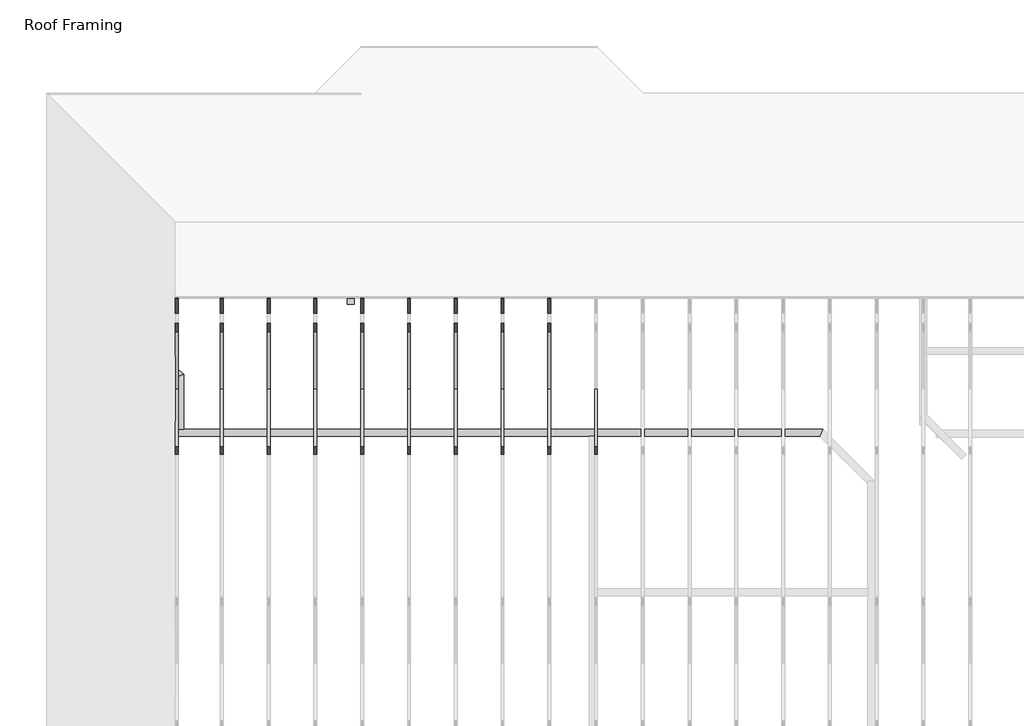
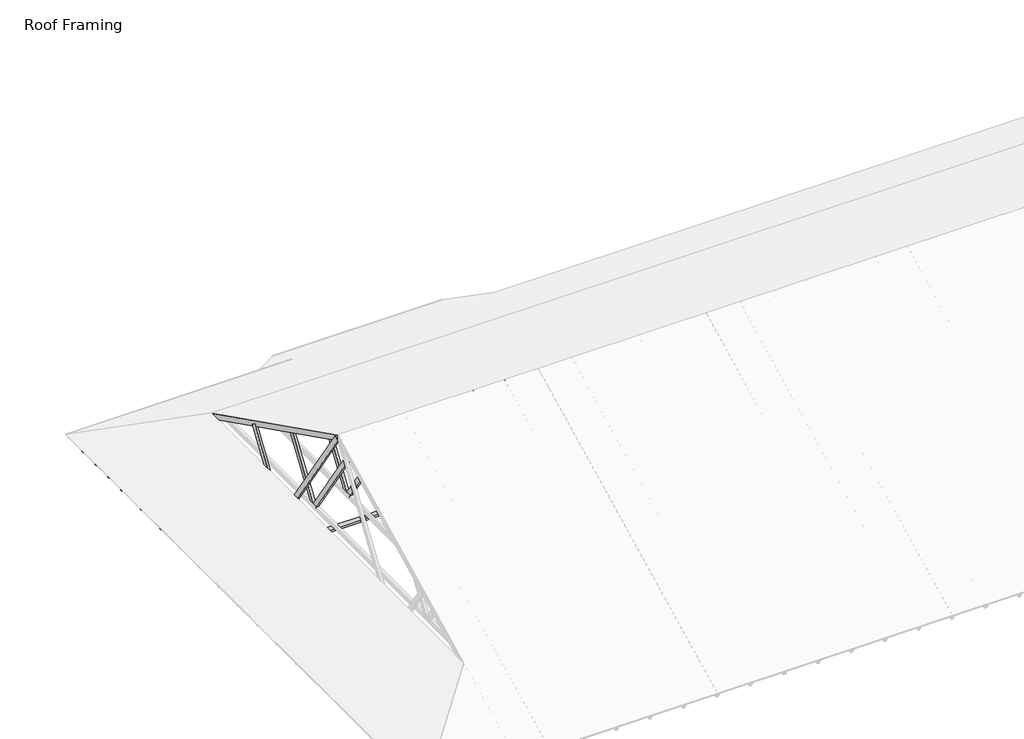
# One storey, part 5 of 7: 46 beams, 19 members.
"""IFC4 building model written with IfcOpenShell, lengths in millimetres."""

import ifcopenshell
import ifcopenshell.guid

model = None  # the IFC model being written
_history = None  # IfcOwnerHistory: only IFC2X3 demands one
_inside = {}  # id of a spatial element -> (the spatial element, [elements in it])
_under = {}  # id of a project, library or spatial element -> (it, [spatial elements below it])
_declared = {}  # id of a project -> (the project, [libraries it declares])
_typed = {}  # id of a type object -> (the type object, [elements of that type])
_made_of = {}  # id of a material, layer set ... -> (it, [elements and type objects made of it])


def new_model(schema):
    """Start an empty IFC model of exactly this schema.

    Asked for "IFC4X3", IfcOpenShell would pick the latest addendum, in which some entities
    have other attributes; the version numbers below select the first issue.
    IFC2X3 requires an IfcOwnerHistory on every rooted entity: one is made here for all.
    """
    global model, _history
    if schema == "IFC4X3":
        model = ifcopenshell.file(schema_version=(4, 3, 0, 0))
    else:
        model = ifcopenshell.file(schema=schema)
    _inside.clear()
    _under.clear()
    _declared.clear()
    _typed.clear()
    _made_of.clear()
    _history = None
    if model.schema == "IFC2X3":
        org = make("IfcOrganization", Name="unknown")
        user = make(
            "IfcPersonAndOrganization",
            ThePerson=make("IfcPerson", FamilyName="unknown"),
            TheOrganization=org,
        )
        app = make(
            "IfcApplication",
            ApplicationDeveloper=org,
            Version="unknown",
            ApplicationFullName="unknown",
            ApplicationIdentifier="unknown",
        )
        _history = make(
            "IfcOwnerHistory",
            OwningUser=user,
            OwningApplication=app,
            ChangeAction="ADDED",
            CreationDate=0,
        )
    return model


def make(cls, **values):
    """One entity of the class cls with the attributes given. An attribute that is None is left unset."""
    return model.create_entity(
        cls, **{name: value for name, value in values.items() if value is not None}
    )


def rooted(cls, **values):
    """An entity with a GlobalId (a new one), such as an element, a storey or a relation."""
    return make(cls, GlobalId=ifcopenshell.guid.new(), OwnerHistory=_history, **values)


def si_unit(unit_type, name, prefix=None):
    """IfcSIUnit, for example si_unit("LENGTHUNIT", "METRE", prefix="MILLI")."""
    return make("IfcSIUnit", UnitType=unit_type, Prefix=prefix, Name=name)


def assignment(units):
    """IfcUnitAssignment: the units of a project."""
    return None if units is None else make("IfcUnitAssignment", Units=units)


def point(xyz):
    """IfcCartesianPoint."""
    return None if xyz is None else make("IfcCartesianPoint", Coordinates=xyz)


def direction(xyz):
    """IfcDirection."""
    return None if xyz is None else make("IfcDirection", DirectionRatios=xyz)


def frame(location, z_axis=None, x_axis=None):
    """IfcAxis2Placement3D, a coordinate frame: its origin and axes. An axis left out is left unset."""
    return make(
        "IfcAxis2Placement3D",
        Location=point(location),
        Axis=direction(z_axis),
        RefDirection=direction(x_axis),
    )


def origin():
    """The frame at (0, 0, 0) with its axes left unset."""
    return frame((0.0, 0.0, 0.0))


def place(relative_to, where):
    """IfcLocalPlacement: puts the frame where relative to a parent placement (None: the world)."""
    return make(
        "IfcLocalPlacement", PlacementRelTo=relative_to, RelativePlacement=where
    )


def context(
    kind, dimensions, precision=None, world=None, true_north=None, identifier=None
):
    """IfcGeometricRepresentationContext, for example the 3D "Model" context."""
    return make(
        "IfcGeometricRepresentationContext",
        ContextIdentifier=identifier,
        ContextType=kind,
        CoordinateSpaceDimension=dimensions,
        Precision=precision,
        WorldCoordinateSystem=world,
        TrueNorth=true_north,
    )


def project(units=None, contexts=None):
    """IfcProject with its units and contexts."""
    return rooted(
        "IfcProject",
        Name="project",
        RepresentationContexts=contexts,
        UnitsInContext=assignment(units),
    )


def spatial(cls, under=None, at=None, **own):
    """A site, building, storey or space (cls), placed at a placement, below another one or the project."""
    s = rooted(cls, ObjectPlacement=at, **own)
    if under is not None:
        _under.setdefault(under.id(), (under, []))[1].append(s)
    return s


def polyline(points):
    """IfcPolyline through the points."""
    return make("IfcPolyline", Points=[point(p) for p in points])


def outline(outer, holes=None, kind="AREA"):
    """IfcArbitraryClosedProfileDef: a profile drawn as a closed curve; with holes, ...WithVoids."""
    if holes is None:
        return make("IfcArbitraryClosedProfileDef", ProfileType=kind, OuterCurve=outer)
    return make(
        "IfcArbitraryProfileDefWithVoids",
        ProfileType=kind,
        OuterCurve=outer,
        InnerCurves=holes,
    )


def extrude(swept, where, along, depth):
    """IfcExtrudedAreaSolid: the profile swept, set in the frame where, extruded along a direction by depth."""
    return make(
        "IfcExtrudedAreaSolid",
        SweptArea=swept,
        Position=where,
        ExtrudedDirection=direction(along),
        Depth=depth,
    )


def shape(context_of_items, identifier, shape_type, items):
    """IfcShapeRepresentation: the items that make up one representation, for example the "Body"."""
    return make(
        "IfcShapeRepresentation",
        ContextOfItems=context_of_items,
        RepresentationIdentifier=identifier,
        RepresentationType=shape_type,
        Items=items,
    )


def source(mapping_origin, context_of_items, identifier, shape_type, items):
    """IfcRepresentationMap: a shape defined once, which mapped items show again and again."""
    return make(
        "IfcRepresentationMap",
        MappingOrigin=mapping_origin,
        MappedRepresentation=shape(context_of_items, identifier, shape_type, items),
    )


def transform(
    local_origin,
    x_axis=None,
    y_axis=None,
    z_axis=None,
    scale=None,
    scale2=None,
    scale3=None,
    uniform=True,
):
    """IfcCartesianTransformationOperator3D, or its non-uniform kind. x_axis, y_axis, z_axis: its Axis1, 2, 3."""
    if uniform:
        return make(
            "IfcCartesianTransformationOperator3D",
            Axis1=direction(x_axis),
            Axis2=direction(y_axis),
            LocalOrigin=point(local_origin),
            Scale=scale,
            Axis3=direction(z_axis),
        )
    return make(
        "IfcCartesianTransformationOperator3DnonUniform",
        Axis1=direction(x_axis),
        Axis2=direction(y_axis),
        LocalOrigin=point(local_origin),
        Scale=scale,
        Axis3=direction(z_axis),
        Scale2=scale2,
        Scale3=scale3,
    )


def mapped(mapping_source, mapping_target):
    """IfcMappedItem: shows the shape of a source again, moved by a transform."""
    return make(
        "IfcMappedItem", MappingSource=mapping_source, MappingTarget=mapping_target
    )


def made_of(thing, what):
    """Note that an element or type object is made of a material, layer set ...; save() writes the relation."""
    if what is not None:
        _made_of.setdefault(what.id(), (what, []))[1].append(thing)
    return thing


def element(
    cls,
    number,
    at=None,
    inside=None,
    cuts=None,
    type_object=None,
    material=None,
    context=None,
    identifier="Body",
    shape_type=None,
    held_by="IfcProductDefinitionShape",
    body=None,
    shapes=None,
    **own,
):
    """One element of the class cls, such as IfcWall. Its Tag is "e" and its number.

    at: its placement. inside: the storey or other place that contains it. cuts: it is an
    opening in that element (IfcRelVoidsElement). A single representation is given by context,
    identifier, shape_type and body (its items); several are given by shapes. held_by: the class
    of the entity that holds the representations. save() writes the other relations.
    """
    e = rooted(cls, Tag="e%d" % number, ObjectPlacement=at, **own)
    if body is not None:
        shapes = [shape(context, identifier, shape_type, body)]
    if shapes is not None:
        e.Representation = make(held_by, Representations=shapes)
    if inside is not None:
        _inside.setdefault(inside.id(), (inside, []))[1].append(e)
    if cuts is not None:
        rooted(
            "IfcRelVoidsElement", RelatingBuildingElement=cuts, RelatedOpeningElement=e
        )
    if type_object is not None:
        _typed.setdefault(type_object.id(), (type_object, []))[1].append(e)
    return made_of(e, material)


def aggregate(whole, parts):
    """IfcRelAggregates: a whole, such as a stair, and the parts it consists of."""
    return rooted("IfcRelAggregates", RelatingObject=whole, RelatedObjects=parts)


def save(model, path):
    """Write the relations noted so far, then the file.

    IfcRelAggregates (storeys below a building ...), IfcRelContainedInSpatialStructure (elements
    in a storey), IfcRelDefinesByType, IfcRelAssociatesMaterial and IfcRelDeclares: one each for
    every whole, place, type object, material and project.
    """
    for whole, parts in _under.values():
        aggregate(whole, parts)
    for where, things in _inside.values():
        rooted(
            "IfcRelContainedInSpatialStructure",
            RelatedElements=things,
            RelatingStructure=where,
        )
    for kind, things in _typed.values():
        rooted("IfcRelDefinesByType", RelatedObjects=things, RelatingType=kind)
    for what, things in _made_of.values():
        rooted("IfcRelAssociatesMaterial", RelatedObjects=things, RelatingMaterial=what)
    for by, libraries in _declared.values():
        rooted("IfcRelDeclares", RelatingContext=by, RelatedDefinitions=libraries)
    model.write(path)


def dimension_lumber_2cac8895(model_context):
    return source(origin(), model_context, "Body", "SweptSolid", [
        extrude(outline(polyline([(1119.2453323, 44.45), (1119.2453323, -44.45), (-1074.7953323, -44.45), (-1074.7953323, 44.45), (1119.2453323, 44.45)])), frame((0.0, 0.0, -19.05), z_axis=(0.0, 0.0, 1.0), x_axis=(1.0, 0.0, 0.0)), (0.0, 0.0, 1.0), 38.1),
    ])


def dimension_lumber_dae2390a(model_context):
    return source(origin(), model_context, "Body", "SweptSolid", [
        extrude(outline(polyline([(120.65, 44.45), (120.65, -44.45), (-3333.75, -44.45), (-3333.75, 44.45), (120.65, 44.45)])), frame((0.0, 0.0, -19.05), z_axis=(0.0, 0.0, 1.0), x_axis=(1.0, 0.0, 0.0)), (0.0, 0.0, 1.0), 38.1),
    ])


def dimension_lumber_0ba03532(model_context):
    return source(origin(), model_context, "Body", "SweptSolid", [
        extrude(outline(polyline([(1590.9128229, 44.45), (1590.9128229, -44.45), (-1571.3871771, -44.45), (-1571.3871771, 44.45), (1590.9128229, 44.45)])), frame((0.0, 0.0, -19.05), z_axis=(0.0, 0.0, 1.0), x_axis=(1.0, 0.0, 0.0)), (0.0, 0.0, 1.0), 38.1),
    ])


def dimension_lumber_2x10_header_exterior_df58e940(model_context):
    return source(origin(), model_context, "Body", "SweptSolid", [
        extrude(outline(polyline([(1646.2375, 19.05), (1646.2375, -19.05), (-1592.2625, -19.05), (-1592.2625, 19.05), (1646.2375, 19.05)])), frame((0.0, 0.0, -117.475), z_axis=(0.0, 0.0, 1.0), x_axis=(1.0, 0.0, 0.0)), (0.0, 0.0, 1.0), 234.95),
    ])


model = new_model("IFC4")

# Units and contexts
model_context = context("Model", 3, world=origin())
ifc_project = project(units=[si_unit("LENGTHUNIT", "METRE", prefix="MILLI")], contexts=[model_context])

# Site, building, storey
site = spatial("IfcSite", under=ifc_project)
building = spatial("IfcBuilding", under=site)
storey = spatial("IfcBuildingStorey", under=building, Name="Roof Framing", Elevation=2768.6)

# Beams
placement = place(None, origin())
element("IfcBeam", 1, ObjectType="Dimension Lumber : Roof Lumbers", at=placement, inside=storey, context=model_context, shape_type="SweptSolid", body=[
    extrude(outline(polyline([(-5032.8152251, 251.1959053), (-5032.8152251, 213.0959053), (-6240.9027251, 213.0959053), (-6240.9027251, 251.1959053), (-5032.8152251, 251.1959053)])), frame((0.0, 0.0, 2768.6), z_axis=(0.0, 0.0, 1.0), x_axis=(1.0, 0.0, 0.0)), (0.0, 0.0, 1.0), 88.9),
    extrude(outline(polyline([(2768.6, -5032.8152251), (2857.5, -5032.8152251), (2857.5, -6064.1385305), (2769.1179027, -6240.9027251), (2768.6, -6240.9027251), (2768.6, -5032.8152251)])), frame((0.0, 213.0959053, 0.0), z_axis=(0.0, 1.0, 0.0), x_axis=(0.0, 0.0, 1.0)), (0.0, 0.0, 1.0), 38.1),
])
element("IfcBeam", 2, ObjectType="Dimension Lumber : Roof Lumbers", at=placement, inside=storey, context=model_context, shape_type="SweptSolid", body=[
    extrude(outline(polyline([(-5032.8152251, 860.7959053), (-5032.8152251, 822.6959053), (-6240.9027251, 822.6959053), (-6240.9027251, 860.7959053), (-5032.8152251, 860.7959053)])), frame((0.0, 0.0, 2768.6), z_axis=(0.0, 0.0, 1.0), x_axis=(1.0, 0.0, 0.0)), (0.0, 0.0, 1.0), 88.9),
    extrude(outline(polyline([(2768.6, -5032.8152251), (2857.5, -5032.8152251), (2857.5, -6064.1385305), (2769.1179027, -6240.9027251), (2768.6, -6240.9027251), (2768.6, -5032.8152251)])), frame((0.0, 822.6959053, 0.0), z_axis=(0.0, 1.0, 0.0), x_axis=(0.0, 0.0, 1.0)), (0.0, 0.0, 1.0), 38.1),
])
element("IfcBeam", 3, ObjectType="Dimension Lumber : Roof Lumbers", at=placement, inside=storey, context=model_context, shape_type="SweptSolid", body=[
    extrude(outline(polyline([(-5032.8152251, 1470.3959053), (-5032.8152251, 1432.2959053), (-6240.9027251, 1432.2959053), (-6240.9027251, 1470.3959053), (-5032.8152251, 1470.3959053)])), frame((0.0, 0.0, 2768.6), z_axis=(0.0, 0.0, 1.0), x_axis=(1.0, 0.0, 0.0)), (0.0, 0.0, 1.0), 88.9),
    extrude(outline(polyline([(2768.6, -5032.8152251), (2857.5, -5032.8152251), (2857.5, -6064.1385305), (2769.1179027, -6240.9027251), (2768.6, -6240.9027251), (2768.6, -5032.8152251)])), frame((0.0, 1432.2959053, 0.0), z_axis=(0.0, 1.0, 0.0), x_axis=(0.0, 0.0, 1.0)), (0.0, 0.0, 1.0), 38.1),
])
element("IfcBeam", 4, ObjectType="Dimension Lumber : Roof Lumbers", at=placement, inside=storey, context=model_context, shape_type="SweptSolid", body=[
    extrude(outline(polyline([(-5032.8152251, 2079.9959053), (-5032.8152251, 2041.8959053), (-6240.9027251, 2041.8959053), (-6240.9027251, 2079.9959053), (-5032.8152251, 2079.9959053)])), frame((0.0, 0.0, 2768.6), z_axis=(0.0, 0.0, 1.0), x_axis=(1.0, 0.0, 0.0)), (0.0, 0.0, 1.0), 88.9),
    extrude(outline(polyline([(2768.6, -5032.8152251), (2857.5, -5032.8152251), (2857.5, -6064.1385305), (2769.1179027, -6240.9027251), (2768.6, -6240.9027251), (2768.6, -5032.8152251)])), frame((0.0, 2041.8959053, 0.0), z_axis=(0.0, 1.0, 0.0), x_axis=(0.0, 0.0, 1.0)), (0.0, 0.0, 1.0), 38.1),
])
element("IfcBeam", 5, ObjectType="Dimension Lumber : Roof Lumbers", at=placement, inside=storey, context=model_context, shape_type="SweptSolid", body=[
    extrude(outline(polyline([(-5032.8152251, 2689.5959053), (-5032.8152251, 2651.4959053), (-6240.9027251, 2651.4959053), (-6240.9027251, 2689.5959053), (-5032.8152251, 2689.5959053)])), frame((0.0, 0.0, 2768.6), z_axis=(0.0, 0.0, 1.0), x_axis=(1.0, 0.0, 0.0)), (0.0, 0.0, 1.0), 88.9),
    extrude(outline(polyline([(2768.6, -5032.8152251), (2857.5, -5032.8152251), (2857.5, -6064.1385305), (2769.1179027, -6240.9027251), (2768.6, -6240.9027251), (2768.6, -5032.8152251)])), frame((0.0, 2651.4959053, 0.0), z_axis=(0.0, 1.0, 0.0), x_axis=(0.0, 0.0, 1.0)), (0.0, 0.0, 1.0), 38.1),
])
element("IfcBeam", 6, ObjectType="Dimension Lumber : Roof Lumbers", at=placement, inside=storey, context=model_context, shape_type="SweptSolid", body=[
    extrude(outline(polyline([(-5032.8152251, 3299.1959053), (-5032.8152251, 3261.0959053), (-6240.9027251, 3261.0959053), (-6240.9027251, 3299.1959053), (-5032.8152251, 3299.1959053)])), frame((0.0, 0.0, 2768.6), z_axis=(0.0, 0.0, 1.0), x_axis=(1.0, 0.0, 0.0)), (0.0, 0.0, 1.0), 88.9),
    extrude(outline(polyline([(2768.6, -5032.8152251), (2857.5, -5032.8152251), (2857.5, -6064.1385305), (2769.1179027, -6240.9027251), (2768.6, -6240.9027251), (2768.6, -5032.8152251)])), frame((0.0, 3261.0959053, 0.0), z_axis=(0.0, 1.0, 0.0), x_axis=(0.0, 0.0, 1.0)), (0.0, 0.0, 1.0), 38.1),
])
element("IfcBeam", 7, ObjectType="Dimension Lumber : Top Supporting Lumbers", at=placement, inside=storey, context=model_context, shape_type="SweptSolid", body=[
    extrude(outline(polyline([(-133.4609188, 5097.8334053), (-133.4609188, 5008.9334053), (-2129.5888108, 5008.9334053), (-2129.5888108, 5097.8334053), (-133.4609188, 5097.8334053)])), frame((0.0, 0.0, 2425.7), z_axis=(0.0, 0.0, 1.0), x_axis=(1.0, 0.0, 0.0)), (0.0, 0.0, 1.0), 38.1),
    extrude(outline(polyline([(-181.7263108, 5008.9334053), (-2129.5888108, 5008.9334053), (-2129.5888108, 5097.8334053), (-144.9027251, 5097.8334053), (-181.7263108, 5008.9334053)])), frame((0.0, 0.0, 2425.7), z_axis=(0.0, 0.0, 1.0), x_axis=(1.0, 0.0, 0.0)), (0.0, 0.0, 1.0), 38.1),
    extrude(outline(polyline([(-181.7263108, 5008.9334053), (-1936.8791394, 5008.9334053), (-1973.7027251, 5097.8334053), (-144.9027251, 5097.8334053), (-181.7263108, 5008.9334053)])), frame((0.0, 0.0, 2425.7), z_axis=(0.0, 0.0, 1.0), x_axis=(1.0, 0.0, 0.0)), (0.0, 0.0, 1.0), 38.1),
])
element("IfcBeam", 8, ObjectType="Dimension Lumber : Top Supporting Lumbers", at=placement, inside=storey, context=model_context, shape_type="SweptSolid", body=[
    extrude(outline(polyline([(-136.9652251, 5097.8334053), (-136.9652251, 5008.9334053), (-1984.8152251, 5008.9334053), (-1984.8152251, 5097.8334053), (-136.9652251, 5097.8334053)])), frame((0.0, 0.0, 2387.6), z_axis=(0.0, 0.0, 1.0), x_axis=(1.0, 0.0, 0.0)), (0.0, 0.0, 1.0), 38.1),
    extrude(outline(polyline([(-136.9652251, 5097.8334053), (-136.9652251, 5008.9334053), (-1936.8791394, 5008.9334053), (-1973.7027251, 5097.8334053), (-136.9652251, 5097.8334053)])), frame((0.0, 0.0, 2387.6), z_axis=(0.0, 0.0, 1.0), x_axis=(1.0, 0.0, 0.0)), (0.0, 0.0, 1.0), 38.1),
    extrude(outline(polyline([(-181.7263108, 5008.9334053), (-1936.8791394, 5008.9334053), (-1973.7027251, 5097.8334053), (-144.9027251, 5097.8334053), (-181.7263108, 5008.9334053)])), frame((0.0, 0.0, 2387.6), z_axis=(0.0, 0.0, 1.0), x_axis=(1.0, 0.0, 0.0)), (0.0, 0.0, 1.0), 38.1),
])
element("IfcBeam", 9, ObjectType="Dimension Lumber : Top Supporting Lumbers", at=placement, inside=storey, context=model_context, shape_type="SweptSolid", body=[
    extrude(outline(polyline([(-2584.7694335, 4361.0431112), (-2647.6312264, 4423.904904), (-1974.0218287, 5097.5143017), (-1911.1600358, 5034.6525089), (-2584.7694335, 4361.0431112)])), frame((0.0, 0.0, 2425.7), z_axis=(0.0, 0.0, 1.0), x_axis=(1.0, 0.0, 0.0)), (0.0, 0.0, 1.0), 38.1),
    extrude(outline(polyline([(-2584.7694335, 4361.0431112), (-2647.6312264, 4423.904904), (-1974.0218287, 5097.5143017), (-1973.2514445, 5096.7439175), (-1936.8791394, 5008.9334053), (-2584.7694335, 4361.0431112)])), frame((0.0, 0.0, 2425.7), z_axis=(0.0, 0.0, 1.0), x_axis=(1.0, 0.0, 0.0)), (0.0, 0.0, 1.0), 38.1),
    extrude(outline(polyline([(-2623.0597276, 4399.3334053), (-2647.6312264, 4423.904904), (-1974.0218287, 5097.5143017), (-1973.2514445, 5096.7439175), (-1936.8791394, 5008.9334053), (-2546.4791394, 4399.3334053), (-2623.0597276, 4399.3334053)])), frame((0.0, 0.0, 2425.7), z_axis=(0.0, 0.0, 1.0), x_axis=(1.0, 0.0, 0.0)), (0.0, 0.0, 1.0), 38.1),
    extrude(outline(polyline([(-2621.4027251, 4450.1334053), (-1974.0218287, 5097.5143017), (-1973.2514445, 5096.7439175), (-1936.8791394, 5008.9334053), (-2546.4791394, 4399.3334053), (-2621.4027251, 4399.3334053), (-2621.4027251, 4450.1334053)])), frame((0.0, 0.0, 2425.7), z_axis=(0.0, 0.0, 1.0), x_axis=(1.0, 0.0, 0.0)), (0.0, 0.0, 1.0), 38.1),
])
element("IfcBeam", 10, ObjectType="Dimension Lumber : Top Supporting Lumbers", at=placement, inside=storey, context=model_context, shape_type="SweptSolid", body=[
    extrude(outline(polyline([(-1969.4575758, 5102.0785546), (-1906.595783, 5039.2167618), (-2584.7694335, 4361.0431112), (-2647.6312264, 4423.904904), (-1969.4575758, 5102.0785546)])), frame((0.0, 0.0, 2387.6), z_axis=(0.0, 0.0, 1.0), x_axis=(1.0, 0.0, 0.0)), (0.0, 0.0, 1.0), 38.1),
    extrude(outline(polyline([(-1936.8791394, 5008.9334053), (-2584.7694335, 4361.0431112), (-2647.6312264, 4423.904904), (-1973.7027251, 5097.8334053), (-1936.8791394, 5008.9334053)])), frame((0.0, 0.0, 2387.6), z_axis=(0.0, 0.0, 1.0), x_axis=(1.0, 0.0, 0.0)), (0.0, 0.0, 1.0), 38.1),
    extrude(outline(polyline([(-1936.8791394, 5008.9334053), (-2546.4791394, 4399.3334053), (-2623.0597276, 4399.3334053), (-2647.6312264, 4423.904904), (-1973.7027251, 5097.8334053), (-1936.8791394, 5008.9334053)])), frame((0.0, 0.0, 2387.6), z_axis=(0.0, 0.0, 1.0), x_axis=(1.0, 0.0, 0.0)), (0.0, 0.0, 1.0), 38.1),
    extrude(outline(polyline([(-1936.8791394, 5008.9334053), (-2546.4791394, 4399.3334053), (-2621.4027251, 4399.3334053), (-2621.4027251, 4450.1334053), (-1973.7027251, 5097.8334053), (-1936.8791394, 5008.9334053)])), frame((0.0, 0.0, 2387.6), z_axis=(0.0, 0.0, 1.0), x_axis=(1.0, 0.0, 0.0)), (0.0, 0.0, 1.0), 38.1),
])
element("IfcBeam", 11, ObjectType="Dimension Lumber : Top Supporting Lumbers", at=placement, inside=storey, context=model_context, shape_type="SweptSolid", body=[
    extrude(outline(polyline([(-5544.0627459, 1818.4935621), (-5576.4196998, 1729.5935621), (-6152.0027251, 1729.5935621), (-6152.0027251, 1818.4935621), (-5544.0627459, 1818.4935621)])), frame((0.0, 0.0, 2692.4), z_axis=(0.0, 0.0, 1.0), x_axis=(1.0, 0.0, 0.0)), (0.0, 0.0, 1.0), 38.1),
])
element("IfcBeam", 12, ObjectType="Dimension Lumber : Top Supporting Lumbers", at=placement, inside=storey, context=model_context, shape_type="SweptSolid", body=[
    extrude(outline(polyline([(-4923.2263621, 1297.5499814), (-5012.1263621, 1256.0952306), (-5576.4196998, 1729.5935621), (-5544.0627459, 1818.4935621), (-4923.2263621, 1297.5499814)])), frame((0.0, 0.0, 2692.4), z_axis=(0.0, 0.0, 1.0), x_axis=(1.0, 0.0, 0.0)), (0.0, 0.0, 1.0), 38.1),
])
element("IfcBeam", 13, ObjectType="Dimension Lumber : Top Supporting Lumbers", at=placement, inside=storey, context=model_context, shape_type="SweptSolid", body=[
    extrude(outline(polyline([(-4923.2263621, 578.2209053), (-5012.1263621, 578.2209053), (-5012.1263621, 1256.0952306), (-4923.2263621, 1297.5499814), (-4923.2263621, 578.2209053)])), frame((0.0, 0.0, 2692.4), z_axis=(0.0, 0.0, 1.0), x_axis=(1.0, 0.0, 0.0)), (0.0, 0.0, 1.0), 38.1),
])
element("IfcBeam", 14, ObjectType="Dimension Lumber : Top Supporting Lumbers", at=placement, inside=storey, context=model_context, shape_type="SweptSolid", body=[
    extrude(outline(polyline([(3409.5097749, 578.2209053), (3372.6861892, 489.3209053), (-6152.0027251, 489.3209053), (-6152.0027251, 578.2209053), (3409.5097749, 578.2209053)])), frame((0.0, 0.0, 2692.4), z_axis=(0.0, 0.0, 1.0), x_axis=(1.0, 0.0, 0.0)), (0.0, 0.0, 1.0), 38.1),
])
dimension_lumber_shape = dimension_lumber_2cac8895(model_context)
element("IfcBeam", 15, ObjectType="Dimension Lumber : Top Supporting Lumbers", at=placement, inside=storey, context=model_context, shape_type="MappedRepresentation", body=[
    mapped(dimension_lumber_shape, transform((-2742.0527251, 3324.538073, 2711.45), x_axis=(0.0, -1.0, 0.0), y_axis=(1.0, 0.0, 0.0), z_axis=(0.0, 0.0, 1.0))),
])
dimension_lumber_2_shape = dimension_lumber_dae2390a(model_context)
element("IfcBeam", 16, ObjectType="Dimension Lumber : Top Supporting Lumbers", at=placement, inside=storey, context=model_context, shape_type="MappedRepresentation", body=[
    mapped(dimension_lumber_2_shape, transform((-2818.2527251, 4443.7834053, 2711.45), x_axis=(1.0, 0.0, 0.0), y_axis=(0.0, 1.0, 0.0), z_axis=(0.0, 0.0, 1.0))),
])
dimension_lumber_3_shape = dimension_lumber_0ba03532(model_context)
element("IfcBeam", 17, ObjectType="Dimension Lumber : Top Supporting Lumbers", at=placement, inside=storey, context=model_context, shape_type="MappedRepresentation", body=[
    mapped(dimension_lumber_3_shape, transform((-1088.115548, 4443.7834053, 2438.796875), x_axis=(1.0, 0.0, 0.0), y_axis=(0.0, 1.0, 0.0), z_axis=(0.0, 0.0, 1.0))),
])
dimension_lumber_2x10_header_exterior_shape = dimension_lumber_2x10_header_exterior_df58e940(model_context)
element("IfcBeam", 18, ObjectType="Dimension Lumber : 2x10 Header Exterior", at=placement, inside=storey, context=model_context, shape_type="MappedRepresentation", body=[
    mapped(dimension_lumber_2x10_header_exterior_shape, transform((-1105.3402251, 4469.1834053, 2651.125), x_axis=(1.0, 0.0, 0.0), y_axis=(0.0, 1.0, 0.0), z_axis=(0.0, 0.0, 1.0))),
])
element("IfcBeam", 19, ObjectType="Dimension Lumber : 2x10 Header Exterior", at=placement, inside=storey, context=model_context, shape_type="MappedRepresentation", body=[
    mapped(dimension_lumber_2x10_header_exterior_shape, transform((-1105.3402251, 4418.3834053, 2651.125), x_axis=(1.0, 0.0, 0.0), y_axis=(0.0, 1.0, 0.0), z_axis=(0.0, 0.0, 1.0))),
])
element("IfcBeam", 20, ObjectType="Dimension Lumber : 2x4 Blocking", at=placement, inside=storey, context=model_context, shape_type="SweptSolid", body=[
    extrude(outline(polyline([(-6671.1152251, 2041.8959053), (-6671.1152251, 2079.9959053), (-6290.1152251, 2079.9959053), (-6290.1152251, 2041.8959053), (-6671.1152251, 2041.8959053)])), frame((0.0, 0.0, 2564.60625), z_axis=(0.0, 0.0, 1.0), x_axis=(1.0, 0.0, 0.0)), (0.0, 0.0, 1.0), 88.9),
    extrude(outline(polyline([(2564.60625, -6649.9260305), (2564.60625, -6290.1152251), (2653.50625, -6290.1152251), (2653.50625, -6472.1260305), (2564.60625, -6649.9260305)])), frame((0.0, 2041.8959053, 0.0), z_axis=(0.0, 1.0, 0.0), x_axis=(0.0, 0.0, 1.0)), (0.0, 0.0, 1.0), 38.1),
])
element("IfcBeam", 21, ObjectType="Dimension Lumber : 2x4 Blocking", at=placement, inside=storey, context=model_context, shape_type="SweptSolid", body=[
    extrude(outline(polyline([(-6671.1152251, 2651.4959053), (-6671.1152251, 2689.5959053), (-6290.1152251, 2689.5959053), (-6290.1152251, 2651.4959053), (-6671.1152251, 2651.4959053)])), frame((0.0, 0.0, 2564.60625), z_axis=(0.0, 0.0, 1.0), x_axis=(1.0, 0.0, 0.0)), (0.0, 0.0, 1.0), 88.9),
    extrude(outline(polyline([(2564.60625, -6649.9260305), (2564.60625, -6290.1152251), (2653.50625, -6290.1152251), (2653.50625, -6472.1260305), (2564.60625, -6649.9260305)])), frame((0.0, 2651.4959053, 0.0), z_axis=(0.0, 1.0, 0.0), x_axis=(0.0, 0.0, 1.0)), (0.0, 0.0, 1.0), 38.1),
])
element("IfcBeam", 22, ObjectType="Dimension Lumber : 2x4 Blocking", at=placement, inside=storey, context=model_context, shape_type="SweptSolid", body=[
    extrude(outline(polyline([(-6671.1152251, 3261.0959053), (-6671.1152251, 3299.1959053), (-6290.1152251, 3299.1959053), (-6290.1152251, 3261.0959053), (-6671.1152251, 3261.0959053)])), frame((0.0, 0.0, 2564.60625), z_axis=(0.0, 0.0, 1.0), x_axis=(1.0, 0.0, 0.0)), (0.0, 0.0, 1.0), 88.9),
    extrude(outline(polyline([(2564.60625, -6649.9260305), (2564.60625, -6290.1152251), (2653.50625, -6290.1152251), (2653.50625, -6472.1260305), (2564.60625, -6649.9260305)])), frame((0.0, 3261.0959053, 0.0), z_axis=(0.0, 1.0, 0.0), x_axis=(0.0, 0.0, 1.0)), (0.0, 0.0, 1.0), 38.1),
])
element("IfcBeam", 23, ObjectType="Dimension Lumber : 2x4 Blocking", at=placement, inside=storey, context=model_context, shape_type="SweptSolid", body=[
    extrude(outline(polyline([(-175.0652251, 5147.0459053), (-175.0652251, 5528.0459053), (-136.9652251, 5528.0459053), (-136.9652251, 5147.0459053), (-175.0652251, 5147.0459053)])), frame((0.0, 0.0, 2259.80625), z_axis=(0.0, 0.0, 1.0), x_axis=(1.0, 0.0, 0.0)), (0.0, 0.0, 1.0), 88.9),
    extrude(outline(polyline([(5147.0459053, 2348.70625), (5329.0567107, 2348.70625), (5506.8567107, 2259.80625), (5147.0459053, 2259.80625), (5147.0459053, 2348.70625)])), frame((-175.0652251, 0.0, 0.0), z_axis=(1.0, 0.0, 0.0), x_axis=(0.0, 1.0, 0.0)), (0.0, 0.0, 1.0), 38.1),
])
element("IfcBeam", 24, ObjectType="Dimension Lumber : 2x4 Blocking", at=placement, inside=storey, context=model_context, shape_type="SweptSolid", body=[
    extrude(outline(polyline([(-784.6652251, 5147.0459053), (-784.6652251, 5528.0459053), (-746.5652251, 5528.0459053), (-746.5652251, 5147.0459053), (-784.6652251, 5147.0459053)])), frame((0.0, 0.0, 2259.80625), z_axis=(0.0, 0.0, 1.0), x_axis=(1.0, 0.0, 0.0)), (0.0, 0.0, 1.0), 88.9),
    extrude(outline(polyline([(5147.0459053, 2348.70625), (5329.0567107, 2348.70625), (5506.8567107, 2259.80625), (5147.0459053, 2259.80625), (5147.0459053, 2348.70625)])), frame((-784.6652251, 0.0, 0.0), z_axis=(1.0, 0.0, 0.0), x_axis=(0.0, 1.0, 0.0)), (0.0, 0.0, 1.0), 38.1),
])
element("IfcBeam", 25, ObjectType="Dimension Lumber : 2x4 Blocking", at=placement, inside=storey, context=model_context, shape_type="SweptSolid", body=[
    extrude(outline(polyline([(-1394.2652251, 5147.0459053), (-1394.2652251, 5528.0459053), (-1356.1652251, 5528.0459053), (-1356.1652251, 5147.0459053), (-1394.2652251, 5147.0459053)])), frame((0.0, 0.0, 2259.80625), z_axis=(0.0, 0.0, 1.0), x_axis=(1.0, 0.0, 0.0)), (0.0, 0.0, 1.0), 88.9),
    extrude(outline(polyline([(5147.0459053, 2348.70625), (5329.0567107, 2348.70625), (5506.8567107, 2259.80625), (5147.0459053, 2259.80625), (5147.0459053, 2348.70625)])), frame((-1394.2652251, 0.0, 0.0), z_axis=(1.0, 0.0, 0.0), x_axis=(0.0, 1.0, 0.0)), (0.0, 0.0, 1.0), 38.1),
])
element("IfcBeam", 26, ObjectType="Dimension Lumber : 2x4 Blocking", at=placement, inside=storey, context=model_context, shape_type="SweptSolid", body=[
    extrude(outline(polyline([(-2003.8652251, 5147.0459053), (-2003.8652251, 5528.0459053), (-1965.7652251, 5528.0459053), (-1965.7652251, 5147.0459053), (-2003.8652251, 5147.0459053)])), frame((0.0, 0.0, 2259.80625), z_axis=(0.0, 0.0, 1.0), x_axis=(1.0, 0.0, 0.0)), (0.0, 0.0, 1.0), 88.9),
    extrude(outline(polyline([(5147.0459053, 2348.70625), (5329.0567107, 2348.70625), (5506.8567107, 2259.80625), (5147.0459053, 2259.80625), (5147.0459053, 2348.70625)])), frame((-2003.8652251, 0.0, 0.0), z_axis=(1.0, 0.0, 0.0), x_axis=(0.0, 1.0, 0.0)), (0.0, 0.0, 1.0), 38.1),
])
element("IfcBeam", 27, ObjectType="Dimension Lumber : 2x4 Blocking", at=placement, inside=storey, context=model_context, shape_type="SweptSolid", body=[
    extrude(outline(polyline([(-2613.4652251, 5147.0459053), (-2613.4652251, 5528.0459053), (-2575.3652251, 5528.0459053), (-2575.3652251, 5147.0459053), (-2613.4652251, 5147.0459053)])), frame((0.0, 0.0, 2259.80625), z_axis=(0.0, 0.0, 1.0), x_axis=(1.0, 0.0, 0.0)), (0.0, 0.0, 1.0), 88.9),
    extrude(outline(polyline([(5147.0459053, 2348.70625), (5329.0567107, 2348.70625), (5506.8567107, 2259.80625), (5147.0459053, 2259.80625), (5147.0459053, 2348.70625)])), frame((-2613.4652251, 0.0, 0.0), z_axis=(1.0, 0.0, 0.0), x_axis=(0.0, 1.0, 0.0)), (0.0, 0.0, 1.0), 38.1),
])
element("IfcBeam", 28, ObjectType="Dimension Lumber : 2x4 Blocking", at=placement, inside=storey, context=model_context, shape_type="SweptSolid", body=[
    extrude(outline(polyline([(-3184.9652251, 4918.4459053), (-3184.9652251, 4537.4459053), (-3223.0652251, 4537.4459053), (-3223.0652251, 4918.4459053), (-3184.9652251, 4918.4459053)])), frame((0.0, 0.0, 2564.60625), z_axis=(0.0, 0.0, 1.0), x_axis=(1.0, 0.0, 0.0)), (0.0, 0.0, 1.0), 88.9),
    extrude(outline(polyline([(4897.2567107, 2564.60625), (4537.4459053, 2564.60625), (4537.4459053, 2653.50625), (4719.4567107, 2653.50625), (4897.2567107, 2564.60625)])), frame((-3223.0652251, 0.0, 0.0), z_axis=(1.0, 0.0, 0.0), x_axis=(0.0, 1.0, 0.0)), (0.0, 0.0, 1.0), 38.1),
])
element("IfcBeam", 29, ObjectType="Dimension Lumber : 2x4 Blocking", at=placement, inside=storey, context=model_context, shape_type="SweptSolid", body=[
    extrude(outline(polyline([(-3794.5652251, 4918.4459053), (-3794.5652251, 4537.4459053), (-3832.6652251, 4537.4459053), (-3832.6652251, 4918.4459053), (-3794.5652251, 4918.4459053)])), frame((0.0, 0.0, 2564.60625), z_axis=(0.0, 0.0, 1.0), x_axis=(1.0, 0.0, 0.0)), (0.0, 0.0, 1.0), 88.9),
    extrude(outline(polyline([(4897.2567107, 2564.60625), (4537.4459053, 2564.60625), (4537.4459053, 2653.50625), (4719.4567107, 2653.50625), (4897.2567107, 2564.60625)])), frame((-3832.6652251, 0.0, 0.0), z_axis=(1.0, 0.0, 0.0), x_axis=(0.0, 1.0, 0.0)), (0.0, 0.0, 1.0), 38.1),
])
element("IfcBeam", 30, ObjectType="Dimension Lumber : 2x4 Blocking", at=placement, inside=storey, context=model_context, shape_type="SweptSolid", body=[
    extrude(outline(polyline([(-4404.1652251, 4918.4459053), (-4404.1652251, 4537.4459053), (-4442.2652251, 4537.4459053), (-4442.2652251, 4918.4459053), (-4404.1652251, 4918.4459053)])), frame((0.0, 0.0, 2564.60625), z_axis=(0.0, 0.0, 1.0), x_axis=(1.0, 0.0, 0.0)), (0.0, 0.0, 1.0), 88.9),
    extrude(outline(polyline([(4897.2567107, 2564.60625), (4537.4459053, 2564.60625), (4537.4459053, 2653.50625), (4719.4567107, 2653.50625), (4897.2567107, 2564.60625)])), frame((-4442.2652251, 0.0, 0.0), z_axis=(1.0, 0.0, 0.0), x_axis=(0.0, 1.0, 0.0)), (0.0, 0.0, 1.0), 38.1),
])
element("IfcBeam", 31, ObjectType="Dimension Lumber : 2x4 Blocking", at=placement, inside=storey, context=model_context, shape_type="SweptSolid", body=[
    extrude(outline(polyline([(-5032.8152251, 4537.4459053), (-5032.8152251, 4918.4459053), (-4994.7152251, 4918.4459053), (-4994.7152251, 4537.4459053), (-5032.8152251, 4537.4459053)])), frame((0.0, 0.0, 2564.60625), z_axis=(0.0, 0.0, 1.0), x_axis=(1.0, 0.0, 0.0)), (0.0, 0.0, 1.0), 88.9),
    extrude(outline(polyline([(4537.4459053, 2653.50625), (4719.4567107, 2653.50625), (4897.2567107, 2564.60625), (4537.4459053, 2564.60625), (4537.4459053, 2653.50625)])), frame((-5032.8152251, 0.0, 0.0), z_axis=(1.0, 0.0, 0.0), x_axis=(0.0, 1.0, 0.0)), (0.0, 0.0, 1.0), 38.1),
])
element("IfcBeam", 32, ObjectType="Dimension Lumber : 2x4 Blocking", at=placement, inside=storey, context=model_context, shape_type="SweptSolid", body=[
    extrude(outline(polyline([(-5458.2652251, 4537.4459053), (-5458.2652251, 4918.4459053), (-5420.1652251, 4918.4459053), (-5420.1652251, 4537.4459053), (-5458.2652251, 4537.4459053)])), frame((0.0, 0.0, 2564.60625), z_axis=(0.0, 0.0, 1.0), x_axis=(1.0, 0.0, 0.0)), (0.0, 0.0, 1.0), 88.9),
    extrude(outline(polyline([(4537.4459053, 2653.50625), (4719.4567107, 2653.50625), (4897.2567107, 2564.60625), (4537.4459053, 2564.60625), (4537.4459053, 2653.50625)])), frame((-5458.2652251, 0.0, 0.0), z_axis=(1.0, 0.0, 0.0), x_axis=(0.0, 1.0, 0.0)), (0.0, 0.0, 1.0), 38.1),
])
element("IfcBeam", 33, ObjectType="Dimension Lumber : 2x4 Blocking", at=placement, inside=storey, context=model_context, shape_type="SweptSolid", body=[
    extrude(outline(polyline([(-5864.6652251, 4537.4459053), (-5864.6652251, 4918.4459053), (-5826.5652251, 4918.4459053), (-5826.5652251, 4537.4459053), (-5864.6652251, 4537.4459053)])), frame((0.0, 0.0, 2564.60625), z_axis=(0.0, 0.0, 1.0), x_axis=(1.0, 0.0, 0.0)), (0.0, 0.0, 1.0), 88.9),
    extrude(outline(polyline([(4537.4459053, 2653.50625), (4719.4567107, 2653.50625), (4897.2567107, 2564.60625), (4537.4459053, 2564.60625), (4537.4459053, 2653.50625)])), frame((-5864.6652251, 0.0, 0.0), z_axis=(1.0, 0.0, 0.0), x_axis=(0.0, 1.0, 0.0)), (0.0, 0.0, 1.0), 38.1),
])
element("IfcBeam", 34, ObjectType="Dimension Lumber : 2x4 Blocking", at=placement, inside=storey, context=model_context, shape_type="SweptSolid", body=[
    extrude(outline(polyline([(-6271.0652251, 4537.4459053), (-6271.0652251, 4918.4459053), (-6232.9652251, 4918.4459053), (-6232.9652251, 4537.4459053), (-6271.0652251, 4537.4459053)])), frame((0.0, 0.0, 2564.60625), z_axis=(0.0, 0.0, 1.0), x_axis=(1.0, 0.0, 0.0)), (0.0, 0.0, 1.0), 88.9),
    extrude(outline(polyline([(4537.4459053, 2653.50625), (4719.4567107, 2653.50625), (4897.2567107, 2564.60625), (4537.4459053, 2564.60625), (4537.4459053, 2653.50625)])), frame((-6271.0652251, 0.0, 0.0), z_axis=(1.0, 0.0, 0.0), x_axis=(0.0, 1.0, 0.0)), (0.0, 0.0, 1.0), 38.1),
])
element("IfcBeam", 35, ObjectType="Dimension Lumber : 2x4 Blocking", at=placement, inside=storey, context=model_context, shape_type="SweptSolid", body=[
    extrude(outline(polyline([(-6671.1152251, 3667.4959053), (-6671.1152251, 3705.5959053), (-6290.1152251, 3705.5959053), (-6290.1152251, 3667.4959053), (-6671.1152251, 3667.4959053)])), frame((0.0, 0.0, 2564.60625), z_axis=(0.0, 0.0, 1.0), x_axis=(1.0, 0.0, 0.0)), (0.0, 0.0, 1.0), 88.9),
    extrude(outline(polyline([(2564.60625, -6649.9260305), (2564.60625, -6290.1152251), (2653.50625, -6290.1152251), (2653.50625, -6472.1260305), (2564.60625, -6649.9260305)])), frame((0.0, 3667.4959053, 0.0), z_axis=(0.0, 1.0, 0.0), x_axis=(0.0, 0.0, 1.0)), (0.0, 0.0, 1.0), 38.1),
])
element("IfcBeam", 36, ObjectType="Dimension Lumber : 2x4 Blocking", at=placement, inside=storey, context=model_context, shape_type="SweptSolid", body=[
    extrude(outline(polyline([(-6671.1152251, 4073.8959053), (-6671.1152251, 4111.9959053), (-6290.1152251, 4111.9959053), (-6290.1152251, 4073.8959053), (-6671.1152251, 4073.8959053)])), frame((0.0, 0.0, 2564.60625), z_axis=(0.0, 0.0, 1.0), x_axis=(1.0, 0.0, 0.0)), (0.0, 0.0, 1.0), 88.9),
    extrude(outline(polyline([(2564.60625, -6649.9260305), (2564.60625, -6290.1152251), (2653.50625, -6290.1152251), (2653.50625, -6472.1260305), (2564.60625, -6649.9260305)])), frame((0.0, 4073.8959053, 0.0), z_axis=(0.0, 1.0, 0.0), x_axis=(0.0, 0.0, 1.0)), (0.0, 0.0, 1.0), 38.1),
])
element("IfcBeam", 37, ObjectType="Dimension Lumber : 2x4 Blocking", at=placement, inside=storey, context=model_context, shape_type="SweptSolid", body=[
    extrude(outline(polyline([(-6671.1152251, 4480.2959053), (-6671.1152251, 4518.3959053), (-6290.1152251, 4518.3959053), (-6290.1152251, 4480.2959053), (-6671.1152251, 4480.2959053)])), frame((0.0, 0.0, 2564.60625), z_axis=(0.0, 0.0, 1.0), x_axis=(1.0, 0.0, 0.0)), (0.0, 0.0, 1.0), 88.9),
    extrude(outline(polyline([(2564.60625, -6649.9260305), (2564.60625, -6290.1152251), (2653.50625, -6290.1152251), (2653.50625, -6472.1260305), (2564.60625, -6649.9260305)])), frame((0.0, 4480.2959053, 0.0), z_axis=(0.0, 1.0, 0.0), x_axis=(0.0, 0.0, 1.0)), (0.0, 0.0, 1.0), 38.1),
])
element("IfcBeam", 38, ObjectType="Dimension Lumber : 2x4 Truss", at=placement, inside=storey, context=model_context, shape_type="SweptSolid", body=[
    extrude(outline(polyline([(4956.5459053, 2634.3548743), (4916.7886167, 2554.840297), (-682.2540947, 5354.3616527), (-682.2540947, 5453.7548743), (4956.5459053, 2634.3548743)])), frame((-175.0652251, 0.0, 0.0), z_axis=(1.0, 0.0, 0.0), x_axis=(0.0, 1.0, 0.0)), (0.0, 0.0, 1.0), 38.1),
])
element("IfcBeam", 39, ObjectType="Dimension Lumber : 2x4 Truss", at=placement, inside=storey, context=model_context, shape_type="SweptSolid", body=[
    extrude(outline(polyline([(4956.5459053, 2634.3548743), (4916.7886167, 2554.840297), (-682.2540947, 5354.3616527), (-682.2540947, 5453.7548743), (4956.5459053, 2634.3548743)])), frame((-784.6652251, 0.0, 0.0), z_axis=(1.0, 0.0, 0.0), x_axis=(0.0, 1.0, 0.0)), (0.0, 0.0, 1.0), 38.1),
])
element("IfcBeam", 40, ObjectType="Dimension Lumber : 2x4 Truss", at=placement, inside=storey, context=model_context, shape_type="SweptSolid", body=[
    extrude(outline(polyline([(4956.5459053, 2634.3548743), (4916.7886167, 2554.840297), (-682.2540947, 5354.3616527), (-682.2540947, 5453.7548743), (4956.5459053, 2634.3548743)])), frame((-1394.2652251, 0.0, 0.0), z_axis=(1.0, 0.0, 0.0), x_axis=(0.0, 1.0, 0.0)), (0.0, 0.0, 1.0), 38.1),
])
element("IfcBeam", 41, ObjectType="Dimension Lumber : 2x4 Truss", at=placement, inside=storey, context=model_context, shape_type="SweptSolid", body=[
    extrude(outline(polyline([(4956.5459053, 2634.3548743), (4916.7886167, 2554.840297), (-682.2540947, 5354.3616527), (-682.2540947, 5453.7548743), (4956.5459053, 2634.3548743)])), frame((-2003.8652251, 0.0, 0.0), z_axis=(1.0, 0.0, 0.0), x_axis=(0.0, 1.0, 0.0)), (0.0, 0.0, 1.0), 38.1),
])
element("IfcBeam", 42, ObjectType="Dimension Lumber : 2x4 Truss", at=placement, inside=storey, context=model_context, shape_type="SweptSolid", body=[
    extrude(outline(polyline([(4956.5459053, 2634.3548743), (4916.7886167, 2554.840297), (-682.2540947, 5354.3616527), (-682.2540947, 5453.7548743), (4956.5459053, 2634.3548743)])), frame((-2613.4652251, 0.0, 0.0), z_axis=(1.0, 0.0, 0.0), x_axis=(0.0, 1.0, 0.0)), (0.0, 0.0, 1.0), 38.1),
])
element("IfcBeam", 43, ObjectType="Dimension Lumber : 2x4 Truss", at=placement, inside=storey, context=model_context, shape_type="SweptSolid", body=[
    extrude(outline(polyline([(4956.5459053, 2634.3548743), (4916.7886167, 2554.840297), (-682.2540947, 5354.3616527), (-682.2540947, 5453.7548743), (4956.5459053, 2634.3548743)])), frame((-3223.0652251, 0.0, 0.0), z_axis=(1.0, 0.0, 0.0), x_axis=(0.0, 1.0, 0.0)), (0.0, 0.0, 1.0), 38.1),
])
element("IfcBeam", 44, ObjectType="Dimension Lumber : 2x4 Truss", at=placement, inside=storey, context=model_context, shape_type="SweptSolid", body=[
    extrude(outline(polyline([(4956.5459053, 2634.3548743), (4916.7886167, 2554.840297), (-682.2540947, 5354.3616527), (-682.2540947, 5453.7548743), (4956.5459053, 2634.3548743)])), frame((-3832.6652251, 0.0, 0.0), z_axis=(1.0, 0.0, 0.0), x_axis=(0.0, 1.0, 0.0)), (0.0, 0.0, 1.0), 38.1),
])
element("IfcBeam", 45, ObjectType="Dimension Lumber : 2x4 Truss", at=placement, inside=storey, context=model_context, shape_type="SweptSolid", body=[
    extrude(outline(polyline([(4956.5459053, 2634.3548743), (4916.7886167, 2554.840297), (-682.2540947, 5354.3616527), (-682.2540947, 5453.7548743), (4956.5459053, 2634.3548743)])), frame((-4442.2652251, 0.0, 0.0), z_axis=(1.0, 0.0, 0.0), x_axis=(0.0, 1.0, 0.0)), (0.0, 0.0, 1.0), 38.1),
])
element("IfcBeam", 46, ObjectType="Dimension Lumber : 2x4 Truss", at=placement, inside=storey, context=model_context, shape_type="SweptSolid", body=[
    extrude(outline(polyline([(4956.5459053, 2634.3548743), (4916.7886167, 2554.840297), (-682.2540947, 5354.3616527), (-682.2540947, 5453.7548743), (4956.5459053, 2634.3548743)])), frame((-5032.8152251, 0.0, 0.0), z_axis=(1.0, 0.0, 0.0), x_axis=(0.0, 1.0, 0.0)), (0.0, 0.0, 1.0), 38.1),
])

# Members
element("IfcMember", 47, ObjectType="Dimension Lumber : 2x4 Truss", at=placement, inside=storey, context=model_context, shape_type="SweptSolid", body=[
    extrude(outline(polyline([(44.45, 19.05), (44.45, -19.05), (-44.45, -19.05), (-44.45, 19.05), (44.45, 19.05)])), frame((453.5847749, 1065.7520094, 2831.7897682), z_axis=(0.0, -0.5576002360134061, 0.8301096173384536), x_axis=(0.0, 0.8301096173384536, 0.5576002360134061)), (0.0, 0.0, 1.0), 3068.6997979),
])
element("IfcMember", 48, ObjectType="Dimension Lumber : 2x4 Truss", at=placement, inside=storey, context=model_context, shape_type="SweptSolid", body=[
    extrude(outline(polyline([(44.45, 19.05), (44.45, -19.05), (-44.45, -19.05), (-44.45, 19.05), (44.45, 19.05)])), frame((-156.0152251, 1065.7520094, 2831.7897682), z_axis=(0.0, -0.5576002360134061, 0.8301096173384536), x_axis=(0.0, 0.8301096173384536, 0.5576002360134061)), (0.0, 0.0, 1.0), 3068.6997979),
])
element("IfcMember", 49, ObjectType="Dimension Lumber : 2x4 Truss", at=placement, inside=storey, context=model_context, shape_type="SweptSolid", body=[
    extrude(outline(polyline([(44.45, -19.05), (-44.45, -19.05), (-44.45, 19.05), (44.45, 19.05), (44.45, -19.05)])), frame((-156.0152251, 1139.5544724, 2831.7982808), z_axis=(0.0, 0.5576002360134061, 0.8301096173384536), x_axis=(0.0, -0.8301096173384536, 0.5576002360134061)), (0.0, 0.0, 1.0), 1484.7518184),
])
element("IfcMember", 50, ObjectType="Dimension Lumber : 2x4 Truss", at=placement, inside=storey, context=model_context, shape_type="SweptSolid", body=[
    extrude(outline(polyline([(44.45, 19.05), (44.45, -19.05), (-44.45, -19.05), (-44.45, 19.05), (44.45, 19.05)])), frame((-765.6152251, 1065.7520094, 2831.7897682), z_axis=(0.0, -0.5576002360134061, 0.8301096173384536), x_axis=(0.0, 0.8301096173384536, 0.5576002360134061)), (0.0, 0.0, 1.0), 3068.6997979),
])
element("IfcMember", 51, ObjectType="Dimension Lumber : 2x4 Truss", at=placement, inside=storey, context=model_context, shape_type="SweptSolid", body=[
    extrude(outline(polyline([(44.45, -19.05), (-44.45, -19.05), (-44.45, 19.05), (44.45, 19.05), (44.45, -19.05)])), frame((-765.6152251, 1139.5544724, 2831.7982808), z_axis=(0.0, 0.5576002360134061, 0.8301096173384536), x_axis=(0.0, -0.8301096173384536, 0.5576002360134061)), (0.0, 0.0, 1.0), 1484.7518184),
])
element("IfcMember", 52, ObjectType="Dimension Lumber : 2x4 Truss", at=placement, inside=storey, context=model_context, shape_type="SweptSolid", body=[
    extrude(outline(polyline([(44.45, 19.05), (44.45, -19.05), (-44.45, -19.05), (-44.45, 19.05), (44.45, 19.05)])), frame((-1375.2152251, 1065.7520094, 2831.7897682), z_axis=(0.0, -0.5576002360134061, 0.8301096173384536), x_axis=(0.0, 0.8301096173384536, 0.5576002360134061)), (0.0, 0.0, 1.0), 3068.6997979),
])
element("IfcMember", 53, ObjectType="Dimension Lumber : 2x4 Truss", at=placement, inside=storey, context=model_context, shape_type="SweptSolid", body=[
    extrude(outline(polyline([(44.45, -19.05), (-44.45, -19.05), (-44.45, 19.05), (44.45, 19.05), (44.45, -19.05)])), frame((-1375.2152251, 1139.5544724, 2831.7982808), z_axis=(0.0, 0.5576002360134061, 0.8301096173384536), x_axis=(0.0, -0.8301096173384536, 0.5576002360134061)), (0.0, 0.0, 1.0), 1484.7518184),
])
element("IfcMember", 54, ObjectType="Dimension Lumber : 2x4 Truss", at=placement, inside=storey, context=model_context, shape_type="SweptSolid", body=[
    extrude(outline(polyline([(44.45, 19.05), (44.45, -19.05), (-44.45, -19.05), (-44.45, 19.05), (44.45, 19.05)])), frame((-1984.8152251, 1065.7520094, 2831.7897682), z_axis=(0.0, -0.5576002360134061, 0.8301096173384536), x_axis=(0.0, 0.8301096173384536, 0.5576002360134061)), (0.0, 0.0, 1.0), 3068.6997979),
])
element("IfcMember", 55, ObjectType="Dimension Lumber : 2x4 Truss", at=placement, inside=storey, context=model_context, shape_type="SweptSolid", body=[
    extrude(outline(polyline([(44.45, -19.05), (-44.45, -19.05), (-44.45, 19.05), (44.45, 19.05), (44.45, -19.05)])), frame((-1984.8152251, 1139.5544724, 2831.7982808), z_axis=(0.0, 0.5576002360134061, 0.8301096173384536), x_axis=(0.0, -0.8301096173384536, 0.5576002360134061)), (0.0, 0.0, 1.0), 1484.7518184),
])
element("IfcMember", 56, ObjectType="Dimension Lumber : 2x4 Truss", at=placement, inside=storey, context=model_context, shape_type="SweptSolid", body=[
    extrude(outline(polyline([(44.45, 19.05), (44.45, -19.05), (-44.45, -19.05), (-44.45, 19.05), (44.45, 19.05)])), frame((-2594.4152251, 1065.7520094, 2831.7897682), z_axis=(0.0, -0.5576002360134061, 0.8301096173384536), x_axis=(0.0, 0.8301096173384536, 0.5576002360134061)), (0.0, 0.0, 1.0), 3068.6997979),
])
element("IfcMember", 57, ObjectType="Dimension Lumber : 2x4 Truss", at=placement, inside=storey, context=model_context, shape_type="SweptSolid", body=[
    extrude(outline(polyline([(44.45, -19.05), (-44.45, -19.05), (-44.45, 19.05), (44.45, 19.05), (44.45, -19.05)])), frame((-2594.4152251, 1139.5544724, 2831.7982808), z_axis=(0.0, 0.5576002360134061, 0.8301096173384536), x_axis=(0.0, -0.8301096173384536, 0.5576002360134061)), (0.0, 0.0, 1.0), 1484.7518184),
])
element("IfcMember", 58, ObjectType="Dimension Lumber : 2x4 Truss", at=placement, inside=storey, context=model_context, shape_type="SweptSolid", body=[
    extrude(outline(polyline([(44.45, 19.05), (44.45, -19.05), (-44.45, -19.05), (-44.45, 19.05), (44.45, 19.05)])), frame((-3204.0152251, 1065.7520094, 2831.7897682), z_axis=(0.0, -0.5576002360134061, 0.8301096173384536), x_axis=(0.0, 0.8301096173384536, 0.5576002360134061)), (0.0, 0.0, 1.0), 3068.6997979),
])
element("IfcMember", 59, ObjectType="Dimension Lumber : 2x4 Truss", at=placement, inside=storey, context=model_context, shape_type="SweptSolid", body=[
    extrude(outline(polyline([(44.45, -19.05), (-44.45, -19.05), (-44.45, 19.05), (44.45, 19.05), (44.45, -19.05)])), frame((-3204.0152251, 1139.5544724, 2831.7982808), z_axis=(0.0, 0.5576002360134061, 0.8301096173384536), x_axis=(0.0, -0.8301096173384536, 0.5576002360134061)), (0.0, 0.0, 1.0), 1484.7518184),
])
element("IfcMember", 60, ObjectType="Dimension Lumber : 2x4 Truss", at=placement, inside=storey, context=model_context, shape_type="SweptSolid", body=[
    extrude(outline(polyline([(44.45, 19.05), (44.45, -19.05), (-44.45, -19.05), (-44.45, 19.05), (44.45, 19.05)])), frame((-3813.6152251, 1065.7520094, 2831.7897682), z_axis=(0.0, -0.5576002360134061, 0.8301096173384536), x_axis=(0.0, 0.8301096173384536, 0.5576002360134061)), (0.0, 0.0, 1.0), 3068.6997979),
])
element("IfcMember", 61, ObjectType="Dimension Lumber : 2x4 Truss", at=placement, inside=storey, context=model_context, shape_type="SweptSolid", body=[
    extrude(outline(polyline([(44.45, -19.05), (-44.45, -19.05), (-44.45, 19.05), (44.45, 19.05), (44.45, -19.05)])), frame((-3813.6152251, 1139.5544724, 2831.7982808), z_axis=(0.0, 0.5576002360134061, 0.8301096173384536), x_axis=(0.0, -0.8301096173384536, 0.5576002360134061)), (0.0, 0.0, 1.0), 1484.7518184),
])
element("IfcMember", 62, ObjectType="Dimension Lumber : 2x4 Truss", at=placement, inside=storey, context=model_context, shape_type="SweptSolid", body=[
    extrude(outline(polyline([(44.45, 19.05), (44.45, -19.05), (-44.45, -19.05), (-44.45, 19.05), (44.45, 19.05)])), frame((-4423.2152251, 1065.7520094, 2831.7897682), z_axis=(0.0, -0.5576002360134061, 0.8301096173384536), x_axis=(0.0, 0.8301096173384536, 0.5576002360134061)), (0.0, 0.0, 1.0), 3068.6997979),
])
element("IfcMember", 63, ObjectType="Dimension Lumber : 2x4 Truss", at=placement, inside=storey, context=model_context, shape_type="SweptSolid", body=[
    extrude(outline(polyline([(44.45, -19.05), (-44.45, -19.05), (-44.45, 19.05), (44.45, 19.05), (44.45, -19.05)])), frame((-4423.2152251, 1139.5544724, 2831.7982808), z_axis=(0.0, 0.5576002360134061, 0.8301096173384536), x_axis=(0.0, -0.8301096173384536, 0.5576002360134061)), (0.0, 0.0, 1.0), 1484.7518184),
])
element("IfcMember", 64, ObjectType="Dimension Lumber : 2x4 Truss", at=placement, inside=storey, context=model_context, shape_type="SweptSolid", body=[
    extrude(outline(polyline([(44.45, 19.05), (44.45, -19.05), (-44.45, -19.05), (-44.45, 19.05), (44.45, 19.05)])), frame((-5013.7652251, 1065.7520094, 2831.7897682), z_axis=(0.0, -0.5576002360134061, 0.8301096173384536), x_axis=(0.0, 0.8301096173384536, 0.5576002360134061)), (0.0, 0.0, 1.0), 3068.6997979),
])
element("IfcMember", 65, ObjectType="Dimension Lumber : 2x4 Truss", at=placement, inside=storey, context=model_context, shape_type="SweptSolid", body=[
    extrude(outline(polyline([(44.45, -19.05), (-44.45, -19.05), (-44.45, 19.05), (44.45, 19.05), (44.45, -19.05)])), frame((-5013.7652251, 1139.5544724, 2831.7982808), z_axis=(0.0, 0.5576002360134061, 0.8301096173384536), x_axis=(0.0, -0.8301096173384536, 0.5576002360134061)), (0.0, 0.0, 1.0), 1484.7518184),
])

save(model, "model.ifc")

# Revit data of these elements
# Type "Dimension Lumber : Roof Lumbers"
#   Assembly Code = "B10"
#   A = 0.0364583 SF
#   Length [instance default] = 5' - 0"
#   b = 0' - 1 1/2"
#   d = 0' - 3 1/2"
#   Structural Material [instance default] = Softwood, Lumber
# Type "Dimension Lumber : Top Supporting Lumbers"
#   Assembly Code = "B10"
#   A = 0.0364583 SF
#   Length [instance default] = 5' - 0"
#   b = 0' - 3 1/2"
#   d = 0' - 1 1/2"
#   Structural Material [instance default] = Softwood, Lumber
# Type "Dimension Lumber : 2x10 Header Exterior"
#   Assembly Code = "B10"
#   A = 0.0963889 SF
#   Length [instance default] = 5' - 0"
#   b = 0' - 1 1/2"
#   d = 0' - 9 1/4"
#   Structural Material [instance default] = Softwood, Lumber
# Type "Dimension Lumber : 2x4 Blocking"
#   Assembly Code = "B10"
#   Cost = 0
#   A = 0.0364583 SF
#   Length [instance default] = 5' - 0"
#   b = 0' - 1 1/2"
#   d = 0' - 3 1/2"
#   Structural Material [instance default] = Softwood, Lumber
# Type "Dimension Lumber : 2x4 Truss"
#   Assembly Code = "B10"
#   Cost = 750
#   A = 0.0364583 SF
#   Length [instance default] = 5' - 0"
#   b = 0' - 1 1/2"
#   d = 0' - 3 1/2"
#   Structural Material [instance default] = Softwood, Lumber
# Elements 1, 2, 3, 4, 5, 6 (IfcBeam, "Dimension Lumber : Roof Lumbers")
#   Comments = ""
#   Structural Material = Douglas Fir #2
#   Phase Created = New Construction
#   Materials on its faces: "Douglas Fir #2"
# Elements 7, 8, 9, 10, 11, 12, 13, 14, 15, 17 (IfcBeam, "Dimension Lumber : Top Supporting Lumbers")
#   Structural Material = Douglas Fir #2
#   Phase Created = New Construction
#   Materials on its faces: "Douglas Fir #2"
# Element 16 (IfcBeam, "Dimension Lumber : Top Supporting Lumbers")
#   Comments = ""
#   Structural Material = Douglas Fir #2
#   Phase Created = New Construction
#   Materials on its faces: "Douglas Fir #2"
# Elements 18, 19 (IfcBeam, "Dimension Lumber : 2x10 Header Exterior")
#   Structural Material = Douglas Fir #2
#   Phase Created = New Construction
#   Materials on its faces: "Douglas Fir #2"
# Elements 20, 21, 22, 23, 24, 25, 26, 27, 28, 29, 30, 31, 32, 33, 34, 35, 36, 37 (IfcBeam, "Dimension Lumber : 2x4 Blocking")
#   Comments = ""
#   Structural Material = Douglas Fir #2
#   Phase Created = New Construction
#   Materials on its faces: "Douglas Fir #2"
# Elements 38, 39, 40, 41, 42, 43, 44, 45, 46 (IfcBeam, "Dimension Lumber : 2x4 Truss")
#   Structural Material = Douglas Fir #2
#   Phase Created = New Construction
#   Materials on its faces: "Douglas Fir #2"
# Elements 47, 48, 49, 50, 51, 52, 53, 54, 55, 56, 57, 58, 59, 60, 61, 62, 63, 64, 65 (IfcMember, "Dimension Lumber : 2x4 Truss")
#   Comments = ""
#   Structural Material = Douglas Fir #2
#   Phase Created = New Construction
#   Materials on its faces: "Douglas Fir #2"
# Materials
#   "Softwood, Lumber": class "Wood", colour RGB 223 192 134, transparency 0, Description = "Pinus Echinata", Cost = 0
#   "Douglas Fir #2": class "Wood", colour RGB 223 192 134, transparency 0, Description = "Pinus Echinata", Cost = 0
